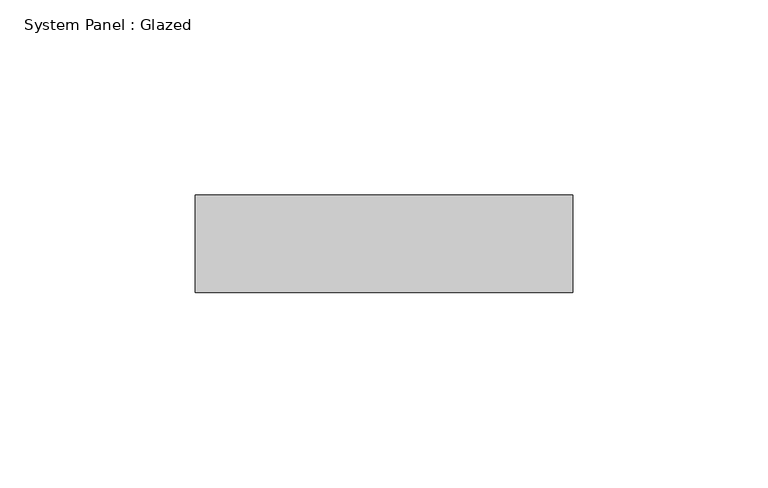
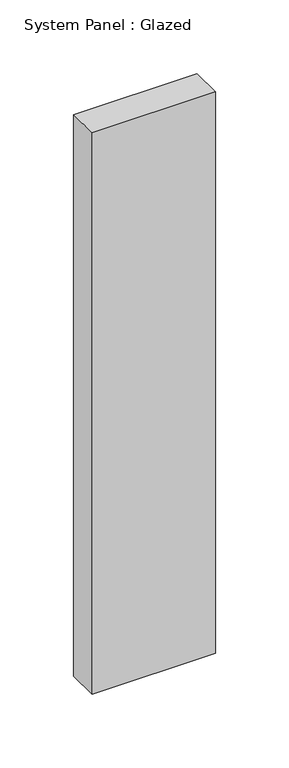
"""IFC4 building model written with IfcOpenShell, lengths in millimetres: plate geometry, System Panel : Glazed."""

from ifc_helpers import new_model, si_unit, origin, origin_with_axes, place, context, project, spatial, polyline, outline, extrude, source, transform, mapped, element, save


def system_panel_glazed_abbeba51(model_context):
    return source(origin(), model_context, "Body", "SweptSolid", [
        extrude(outline(polyline([(48.4090908, 24.5), (-48.4090908, 24.5), (-48.4090908, 49.5), (48.4090908, 49.5), (48.4090908, 24.5)])), origin_with_axes(), (0.0, 0.0, 1.0), 465.0),
    ])


if __name__ == "__main__":
    model = new_model("IFC4")
    model_context = context("Model", 3, world=origin())
    ifc_project = project(units=[si_unit("LENGTHUNIT", "METRE", prefix="MILLI")], contexts=[model_context])
    site = spatial("IfcSite", under=ifc_project)
    building = spatial("IfcBuilding", under=site)
    placement = place(None, origin())
    system_panel_glazed_shape = system_panel_glazed_abbeba51(model_context)
    element("IfcPlate", 1, ObjectType="System Panel : Glazed", at=placement, inside=building, context=model_context, shape_type="MappedRepresentation", body=[
        mapped(system_panel_glazed_shape, transform((0.0, 0.0, 0.0), x_axis=(1.0, 0.0, 0.0), y_axis=(0.0, 1.0, 0.0), z_axis=(0.0, 0.0, 1.0))),
    ])
    save(model, "model.ifc")

# Revit data of these elements
# Element 1 (IfcPlate, "System Panel : Glazed")
#   Materials on its faces: "Glass"
# Materials
#   "Glass": class "Glass", colour RGB 218 227 224, transparency 0.85, Description = "Soda Lime Glass", Cost = 0
